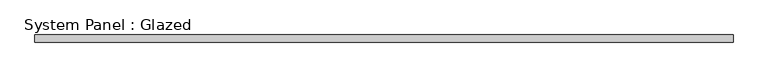
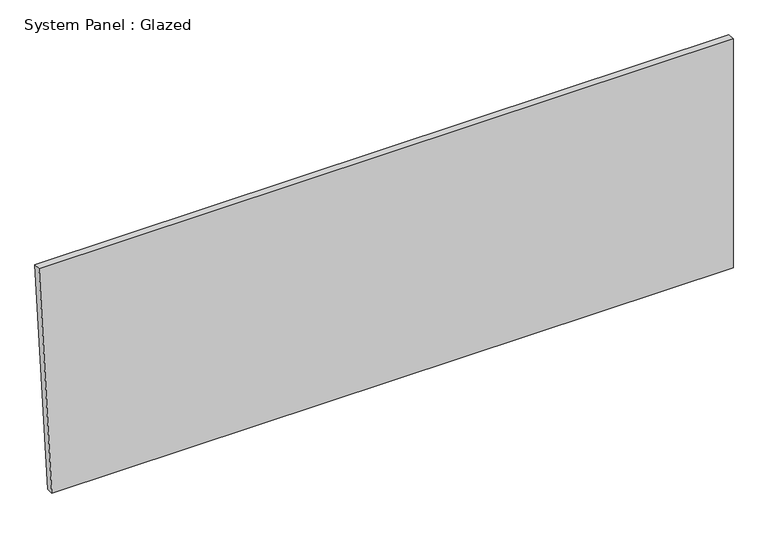
"""IFC4 building model written with IfcOpenShell, lengths in millimetres: plate geometry, System Panel : Glazed."""

import ifcopenshell
import ifcopenshell.guid

model = None  # the IFC model being written
_history = None  # IfcOwnerHistory: only IFC2X3 demands one
_inside = {}  # id of a spatial element -> (the spatial element, [elements in it])
_under = {}  # id of a project, library or spatial element -> (it, [spatial elements below it])
_declared = {}  # id of a project -> (the project, [libraries it declares])
_typed = {}  # id of a type object -> (the type object, [elements of that type])
_made_of = {}  # id of a material, layer set ... -> (it, [elements and type objects made of it])


def new_model(schema):
    """Start an empty IFC model of exactly this schema.

    Asked for "IFC4X3", IfcOpenShell would pick the latest addendum, in which some entities
    have other attributes; the version numbers below select the first issue.
    IFC2X3 requires an IfcOwnerHistory on every rooted entity: one is made here for all.
    """
    global model, _history
    if schema == "IFC4X3":
        model = ifcopenshell.file(schema_version=(4, 3, 0, 0))
    else:
        model = ifcopenshell.file(schema=schema)
    _inside.clear()
    _under.clear()
    _declared.clear()
    _typed.clear()
    _made_of.clear()
    _history = None
    if model.schema == "IFC2X3":
        org = make("IfcOrganization", Name="unknown")
        user = make(
            "IfcPersonAndOrganization",
            ThePerson=make("IfcPerson", FamilyName="unknown"),
            TheOrganization=org,
        )
        app = make(
            "IfcApplication",
            ApplicationDeveloper=org,
            Version="unknown",
            ApplicationFullName="unknown",
            ApplicationIdentifier="unknown",
        )
        _history = make(
            "IfcOwnerHistory",
            OwningUser=user,
            OwningApplication=app,
            ChangeAction="ADDED",
            CreationDate=0,
        )
    return model


def make(cls, **values):
    """One entity of the class cls with the attributes given. An attribute that is None is left unset."""
    return model.create_entity(
        cls, **{name: value for name, value in values.items() if value is not None}
    )


def rooted(cls, **values):
    """An entity with a GlobalId (a new one), such as an element, a storey or a relation."""
    return make(cls, GlobalId=ifcopenshell.guid.new(), OwnerHistory=_history, **values)


def si_unit(unit_type, name, prefix=None):
    """IfcSIUnit, for example si_unit("LENGTHUNIT", "METRE", prefix="MILLI")."""
    return make("IfcSIUnit", UnitType=unit_type, Prefix=prefix, Name=name)


def assignment(units):
    """IfcUnitAssignment: the units of a project."""
    return None if units is None else make("IfcUnitAssignment", Units=units)


def point(xyz):
    """IfcCartesianPoint."""
    return None if xyz is None else make("IfcCartesianPoint", Coordinates=xyz)


def direction(xyz):
    """IfcDirection."""
    return None if xyz is None else make("IfcDirection", DirectionRatios=xyz)


def frame(location, z_axis=None, x_axis=None):
    """IfcAxis2Placement3D, a coordinate frame: its origin and axes. An axis left out is left unset."""
    return make(
        "IfcAxis2Placement3D",
        Location=point(location),
        Axis=direction(z_axis),
        RefDirection=direction(x_axis),
    )


def origin():
    """The frame at (0, 0, 0) with its axes left unset."""
    return frame((0.0, 0.0, 0.0))


def place(relative_to, where):
    """IfcLocalPlacement: puts the frame where relative to a parent placement (None: the world)."""
    return make(
        "IfcLocalPlacement", PlacementRelTo=relative_to, RelativePlacement=where
    )


def context(
    kind, dimensions, precision=None, world=None, true_north=None, identifier=None
):
    """IfcGeometricRepresentationContext, for example the 3D "Model" context."""
    return make(
        "IfcGeometricRepresentationContext",
        ContextIdentifier=identifier,
        ContextType=kind,
        CoordinateSpaceDimension=dimensions,
        Precision=precision,
        WorldCoordinateSystem=world,
        TrueNorth=true_north,
    )


def project(units=None, contexts=None):
    """IfcProject with its units and contexts."""
    return rooted(
        "IfcProject",
        Name="project",
        RepresentationContexts=contexts,
        UnitsInContext=assignment(units),
    )


def spatial(cls, under=None, at=None, **own):
    """A site, building, storey or space (cls), placed at a placement, below another one or the project."""
    s = rooted(cls, ObjectPlacement=at, **own)
    if under is not None:
        _under.setdefault(under.id(), (under, []))[1].append(s)
    return s


def polyline(points):
    """IfcPolyline through the points."""
    return make("IfcPolyline", Points=[point(p) for p in points])


def outline(outer, holes=None, kind="AREA"):
    """IfcArbitraryClosedProfileDef: a profile drawn as a closed curve; with holes, ...WithVoids."""
    if holes is None:
        return make("IfcArbitraryClosedProfileDef", ProfileType=kind, OuterCurve=outer)
    return make(
        "IfcArbitraryProfileDefWithVoids",
        ProfileType=kind,
        OuterCurve=outer,
        InnerCurves=holes,
    )


def extrude(swept, where, along, depth):
    """IfcExtrudedAreaSolid: the profile swept, set in the frame where, extruded along a direction by depth."""
    return make(
        "IfcExtrudedAreaSolid",
        SweptArea=swept,
        Position=where,
        ExtrudedDirection=direction(along),
        Depth=depth,
    )


def shape(context_of_items, identifier, shape_type, items):
    """IfcShapeRepresentation: the items that make up one representation, for example the "Body"."""
    return make(
        "IfcShapeRepresentation",
        ContextOfItems=context_of_items,
        RepresentationIdentifier=identifier,
        RepresentationType=shape_type,
        Items=items,
    )


def source(mapping_origin, context_of_items, identifier, shape_type, items):
    """IfcRepresentationMap: a shape defined once, which mapped items show again and again."""
    return make(
        "IfcRepresentationMap",
        MappingOrigin=mapping_origin,
        MappedRepresentation=shape(context_of_items, identifier, shape_type, items),
    )


def transform(
    local_origin,
    x_axis=None,
    y_axis=None,
    z_axis=None,
    scale=None,
    scale2=None,
    scale3=None,
    uniform=True,
):
    """IfcCartesianTransformationOperator3D, or its non-uniform kind. x_axis, y_axis, z_axis: its Axis1, 2, 3."""
    if uniform:
        return make(
            "IfcCartesianTransformationOperator3D",
            Axis1=direction(x_axis),
            Axis2=direction(y_axis),
            LocalOrigin=point(local_origin),
            Scale=scale,
            Axis3=direction(z_axis),
        )
    return make(
        "IfcCartesianTransformationOperator3DnonUniform",
        Axis1=direction(x_axis),
        Axis2=direction(y_axis),
        LocalOrigin=point(local_origin),
        Scale=scale,
        Axis3=direction(z_axis),
        Scale2=scale2,
        Scale3=scale3,
    )


def mapped(mapping_source, mapping_target):
    """IfcMappedItem: shows the shape of a source again, moved by a transform."""
    return make(
        "IfcMappedItem", MappingSource=mapping_source, MappingTarget=mapping_target
    )


def made_of(thing, what):
    """Note that an element or type object is made of a material, layer set ...; save() writes the relation."""
    if what is not None:
        _made_of.setdefault(what.id(), (what, []))[1].append(thing)
    return thing


def element(
    cls,
    number,
    at=None,
    inside=None,
    cuts=None,
    type_object=None,
    material=None,
    context=None,
    identifier="Body",
    shape_type=None,
    held_by="IfcProductDefinitionShape",
    body=None,
    shapes=None,
    **own,
):
    """One element of the class cls, such as IfcWall. Its Tag is "e" and its number.

    at: its placement. inside: the storey or other place that contains it. cuts: it is an
    opening in that element (IfcRelVoidsElement). A single representation is given by context,
    identifier, shape_type and body (its items); several are given by shapes. held_by: the class
    of the entity that holds the representations. save() writes the other relations.
    """
    e = rooted(cls, Tag="e%d" % number, ObjectPlacement=at, **own)
    if body is not None:
        shapes = [shape(context, identifier, shape_type, body)]
    if shapes is not None:
        e.Representation = make(held_by, Representations=shapes)
    if inside is not None:
        _inside.setdefault(inside.id(), (inside, []))[1].append(e)
    if cuts is not None:
        rooted(
            "IfcRelVoidsElement", RelatingBuildingElement=cuts, RelatedOpeningElement=e
        )
    if type_object is not None:
        _typed.setdefault(type_object.id(), (type_object, []))[1].append(e)
    return made_of(e, material)


def aggregate(whole, parts):
    """IfcRelAggregates: a whole, such as a stair, and the parts it consists of."""
    return rooted("IfcRelAggregates", RelatingObject=whole, RelatedObjects=parts)


def save(model, path):
    """Write the relations noted so far, then the file.

    IfcRelAggregates (storeys below a building ...), IfcRelContainedInSpatialStructure (elements
    in a storey), IfcRelDefinesByType, IfcRelAssociatesMaterial and IfcRelDeclares: one each for
    every whole, place, type object, material and project.
    """
    for whole, parts in _under.values():
        aggregate(whole, parts)
    for where, things in _inside.values():
        rooted(
            "IfcRelContainedInSpatialStructure",
            RelatedElements=things,
            RelatingStructure=where,
        )
    for kind, things in _typed.values():
        rooted("IfcRelDefinesByType", RelatedObjects=things, RelatingType=kind)
    for what, things in _made_of.values():
        rooted("IfcRelAssociatesMaterial", RelatedObjects=things, RelatingMaterial=what)
    for by, libraries in _declared.values():
        rooted("IfcRelDeclares", RelatingContext=by, RelatedDefinitions=libraries)
    model.write(path)


def system_panel_glazed_f82295e9(model_context):
    return source(origin(), model_context, "Body", "SweptSolid", [
        extrude(outline(polyline([(0.0, -1197.3859051), (0.0, 1242.7131117), (866.081558, 1242.7131117), (866.081558, -1242.7131117), (0.0, -1197.3859051)])), frame((0.0, -44.45, 0.0), z_axis=(0.0, 1.0, 0.0), x_axis=(0.0, 0.0, 1.0)), (0.0, 0.0, 1.0), 25.4),
    ])


if __name__ == "__main__":
    model = new_model("IFC4")
    model_context = context("Model", 3, world=origin())
    ifc_project = project(units=[si_unit("LENGTHUNIT", "METRE", prefix="MILLI")], contexts=[model_context])
    site = spatial("IfcSite", under=ifc_project)
    building = spatial("IfcBuilding", under=site)
    placement = place(None, origin())
    system_panel_glazed_shape = system_panel_glazed_f82295e9(model_context)
    element("IfcPlate", 1, ObjectType="System Panel : Glazed", at=placement, inside=building, context=model_context, shape_type="MappedRepresentation", body=[
        mapped(system_panel_glazed_shape, transform((0.0, 0.0, 0.0), x_axis=(1.0, 0.0, 0.0), y_axis=(0.0, 1.0, 0.0), z_axis=(0.0, 0.0, 1.0))),
    ])
    save(model, "model.ifc")

# Revit data of these elements
# Type "System Panel : Glazed"
#   Construction Type Id = "GSP4R"
#   Analytic Construction = "1/8 in Pilkington single glazing"
#   Visual Light Transmittance = 0.9
#   Solar Heat Gain Coefficient = 0.86
#   Heat Transfer Coefficient (U) = 1.18115 BTU/(h·ft²·°F)
#   Define Thermal Properties by = 1
# Element 1 (IfcPlate, "System Panel : Glazed")
#   Materials on its faces: "Glass"
# Materials
#   "Glass": class "Glass", colour RGB 0 128 192, transparency 0.75, Description = "Soda Lime Glass", Cost = 0
